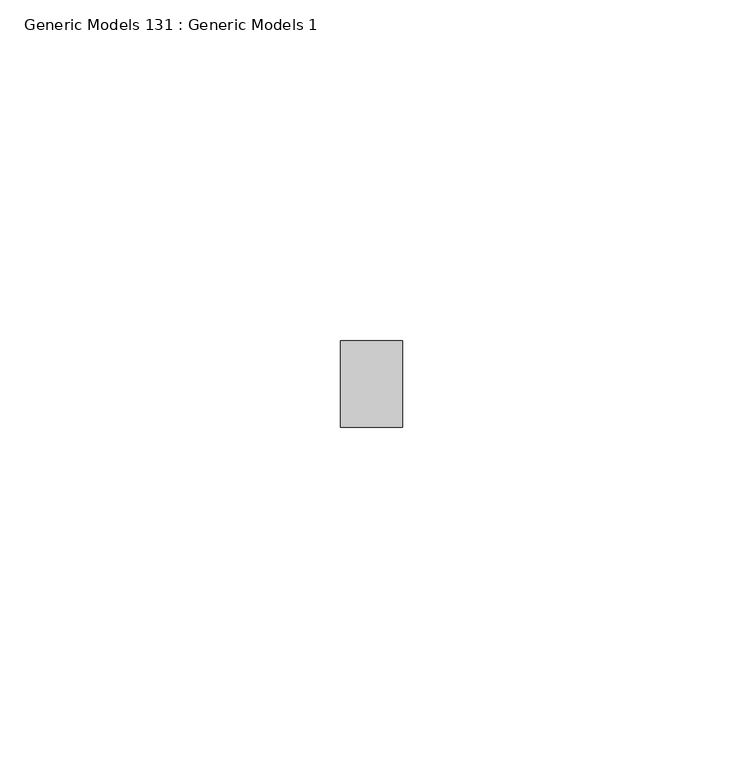
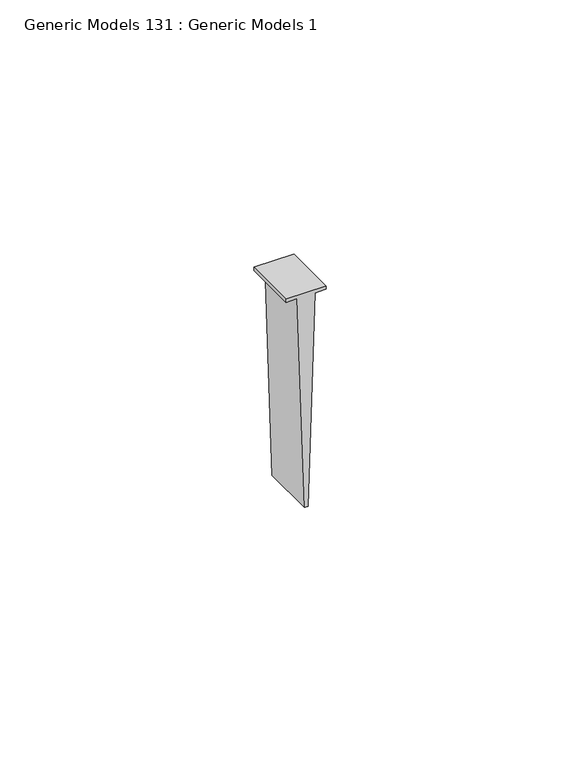
"""IFC4 building model written with IfcOpenShell, lengths in millimetres: proxy geometry, Generic Models 131 : Generic Models 1."""

import ifcopenshell
import ifcopenshell.guid

model = None  # the IFC model being written
_history = None  # IfcOwnerHistory: only IFC2X3 demands one
_inside = {}  # id of a spatial element -> (the spatial element, [elements in it])
_under = {}  # id of a project, library or spatial element -> (it, [spatial elements below it])
_declared = {}  # id of a project -> (the project, [libraries it declares])
_typed = {}  # id of a type object -> (the type object, [elements of that type])
_made_of = {}  # id of a material, layer set ... -> (it, [elements and type objects made of it])


def new_model(schema):
    """Start an empty IFC model of exactly this schema.

    Asked for "IFC4X3", IfcOpenShell would pick the latest addendum, in which some entities
    have other attributes; the version numbers below select the first issue.
    IFC2X3 requires an IfcOwnerHistory on every rooted entity: one is made here for all.
    """
    global model, _history
    if schema == "IFC4X3":
        model = ifcopenshell.file(schema_version=(4, 3, 0, 0))
    else:
        model = ifcopenshell.file(schema=schema)
    _inside.clear()
    _under.clear()
    _declared.clear()
    _typed.clear()
    _made_of.clear()
    _history = None
    if model.schema == "IFC2X3":
        org = make("IfcOrganization", Name="unknown")
        user = make(
            "IfcPersonAndOrganization",
            ThePerson=make("IfcPerson", FamilyName="unknown"),
            TheOrganization=org,
        )
        app = make(
            "IfcApplication",
            ApplicationDeveloper=org,
            Version="unknown",
            ApplicationFullName="unknown",
            ApplicationIdentifier="unknown",
        )
        _history = make(
            "IfcOwnerHistory",
            OwningUser=user,
            OwningApplication=app,
            ChangeAction="ADDED",
            CreationDate=0,
        )
    return model


def make(cls, **values):
    """One entity of the class cls with the attributes given. An attribute that is None is left unset."""
    return model.create_entity(
        cls, **{name: value for name, value in values.items() if value is not None}
    )


def rooted(cls, **values):
    """An entity with a GlobalId (a new one), such as an element, a storey or a relation."""
    return make(cls, GlobalId=ifcopenshell.guid.new(), OwnerHistory=_history, **values)


def si_unit(unit_type, name, prefix=None):
    """IfcSIUnit, for example si_unit("LENGTHUNIT", "METRE", prefix="MILLI")."""
    return make("IfcSIUnit", UnitType=unit_type, Prefix=prefix, Name=name)


def assignment(units):
    """IfcUnitAssignment: the units of a project."""
    return None if units is None else make("IfcUnitAssignment", Units=units)


def point(xyz):
    """IfcCartesianPoint."""
    return None if xyz is None else make("IfcCartesianPoint", Coordinates=xyz)


def direction(xyz):
    """IfcDirection."""
    return None if xyz is None else make("IfcDirection", DirectionRatios=xyz)


def frame(location, z_axis=None, x_axis=None):
    """IfcAxis2Placement3D, a coordinate frame: its origin and axes. An axis left out is left unset."""
    return make(
        "IfcAxis2Placement3D",
        Location=point(location),
        Axis=direction(z_axis),
        RefDirection=direction(x_axis),
    )


def origin():
    """The frame at (0, 0, 0) with its axes left unset."""
    return frame((0.0, 0.0, 0.0))


def place(relative_to, where):
    """IfcLocalPlacement: puts the frame where relative to a parent placement (None: the world)."""
    return make(
        "IfcLocalPlacement", PlacementRelTo=relative_to, RelativePlacement=where
    )


def context(
    kind, dimensions, precision=None, world=None, true_north=None, identifier=None
):
    """IfcGeometricRepresentationContext, for example the 3D "Model" context."""
    return make(
        "IfcGeometricRepresentationContext",
        ContextIdentifier=identifier,
        ContextType=kind,
        CoordinateSpaceDimension=dimensions,
        Precision=precision,
        WorldCoordinateSystem=world,
        TrueNorth=true_north,
    )


def project(units=None, contexts=None):
    """IfcProject with its units and contexts."""
    return rooted(
        "IfcProject",
        Name="project",
        RepresentationContexts=contexts,
        UnitsInContext=assignment(units),
    )


def spatial(cls, under=None, at=None, **own):
    """A site, building, storey or space (cls), placed at a placement, below another one or the project."""
    s = rooted(cls, ObjectPlacement=at, **own)
    if under is not None:
        _under.setdefault(under.id(), (under, []))[1].append(s)
    return s


def polyline(points):
    """IfcPolyline through the points."""
    return make("IfcPolyline", Points=[point(p) for p in points])


def outline(outer, holes=None, kind="AREA"):
    """IfcArbitraryClosedProfileDef: a profile drawn as a closed curve; with holes, ...WithVoids."""
    if holes is None:
        return make("IfcArbitraryClosedProfileDef", ProfileType=kind, OuterCurve=outer)
    return make(
        "IfcArbitraryProfileDefWithVoids",
        ProfileType=kind,
        OuterCurve=outer,
        InnerCurves=holes,
    )


def extrude(swept, where, along, depth):
    """IfcExtrudedAreaSolid: the profile swept, set in the frame where, extruded along a direction by depth."""
    return make(
        "IfcExtrudedAreaSolid",
        SweptArea=swept,
        Position=where,
        ExtrudedDirection=direction(along),
        Depth=depth,
    )


def shape(context_of_items, identifier, shape_type, items):
    """IfcShapeRepresentation: the items that make up one representation, for example the "Body"."""
    return make(
        "IfcShapeRepresentation",
        ContextOfItems=context_of_items,
        RepresentationIdentifier=identifier,
        RepresentationType=shape_type,
        Items=items,
    )


def source(mapping_origin, context_of_items, identifier, shape_type, items):
    """IfcRepresentationMap: a shape defined once, which mapped items show again and again."""
    return make(
        "IfcRepresentationMap",
        MappingOrigin=mapping_origin,
        MappedRepresentation=shape(context_of_items, identifier, shape_type, items),
    )


def transform(
    local_origin,
    x_axis=None,
    y_axis=None,
    z_axis=None,
    scale=None,
    scale2=None,
    scale3=None,
    uniform=True,
):
    """IfcCartesianTransformationOperator3D, or its non-uniform kind. x_axis, y_axis, z_axis: its Axis1, 2, 3."""
    if uniform:
        return make(
            "IfcCartesianTransformationOperator3D",
            Axis1=direction(x_axis),
            Axis2=direction(y_axis),
            LocalOrigin=point(local_origin),
            Scale=scale,
            Axis3=direction(z_axis),
        )
    return make(
        "IfcCartesianTransformationOperator3DnonUniform",
        Axis1=direction(x_axis),
        Axis2=direction(y_axis),
        LocalOrigin=point(local_origin),
        Scale=scale,
        Axis3=direction(z_axis),
        Scale2=scale2,
        Scale3=scale3,
    )


def mapped(mapping_source, mapping_target):
    """IfcMappedItem: shows the shape of a source again, moved by a transform."""
    return make(
        "IfcMappedItem", MappingSource=mapping_source, MappingTarget=mapping_target
    )


def made_of(thing, what):
    """Note that an element or type object is made of a material, layer set ...; save() writes the relation."""
    if what is not None:
        _made_of.setdefault(what.id(), (what, []))[1].append(thing)
    return thing


def element(
    cls,
    number,
    at=None,
    inside=None,
    cuts=None,
    type_object=None,
    material=None,
    context=None,
    identifier="Body",
    shape_type=None,
    held_by="IfcProductDefinitionShape",
    body=None,
    shapes=None,
    **own,
):
    """One element of the class cls, such as IfcWall. Its Tag is "e" and its number.

    at: its placement. inside: the storey or other place that contains it. cuts: it is an
    opening in that element (IfcRelVoidsElement). A single representation is given by context,
    identifier, shape_type and body (its items); several are given by shapes. held_by: the class
    of the entity that holds the representations. save() writes the other relations.
    """
    e = rooted(cls, Tag="e%d" % number, ObjectPlacement=at, **own)
    if body is not None:
        shapes = [shape(context, identifier, shape_type, body)]
    if shapes is not None:
        e.Representation = make(held_by, Representations=shapes)
    if inside is not None:
        _inside.setdefault(inside.id(), (inside, []))[1].append(e)
    if cuts is not None:
        rooted(
            "IfcRelVoidsElement", RelatingBuildingElement=cuts, RelatedOpeningElement=e
        )
    if type_object is not None:
        _typed.setdefault(type_object.id(), (type_object, []))[1].append(e)
    return made_of(e, material)


def aggregate(whole, parts):
    """IfcRelAggregates: a whole, such as a stair, and the parts it consists of."""
    return rooted("IfcRelAggregates", RelatingObject=whole, RelatedObjects=parts)


def save(model, path):
    """Write the relations noted so far, then the file.

    IfcRelAggregates (storeys below a building ...), IfcRelContainedInSpatialStructure (elements
    in a storey), IfcRelDefinesByType, IfcRelAssociatesMaterial and IfcRelDeclares: one each for
    every whole, place, type object, material and project.
    """
    for whole, parts in _under.values():
        aggregate(whole, parts)
    for where, things in _inside.values():
        rooted(
            "IfcRelContainedInSpatialStructure",
            RelatedElements=things,
            RelatingStructure=where,
        )
    for kind, things in _typed.values():
        rooted("IfcRelDefinesByType", RelatedObjects=things, RelatingType=kind)
    for what, things in _made_of.values():
        rooted("IfcRelAssociatesMaterial", RelatedObjects=things, RelatingMaterial=what)
    for by, libraries in _declared.values():
        rooted("IfcRelDeclares", RelatingContext=by, RelatedDefinitions=libraries)
    model.write(path)


def generic_models_131_generic_models_1_dfd9233a(model_context):
    return source(origin(), model_context, "Body", "SweptSolid", [
        extrude(outline(polyline([(-223.594817, 46885.2894531), (-224.388567, 46885.2894531), (-224.388567, 46887.8393167), (-275.188567, 46889.4367058), (-275.188567, 46890.2354003), (-224.388567, 46891.8327895), (-224.388567, 46894.3826531), (-223.594817, 46894.3826531), (-223.594817, 46885.2894531)])), frame((0.0, 565.15, 0.0), z_axis=(0.0, 1.0, 0.0), x_axis=(0.0, 0.0, 1.0)), (0.0, 0.0, 1.0), 12.7),
    ])


if __name__ == "__main__":
    model = new_model("IFC4")
    model_context = context("Model", 3, world=origin())
    ifc_project = project(units=[si_unit("LENGTHUNIT", "METRE", prefix="MILLI")], contexts=[model_context])
    site = spatial("IfcSite", under=ifc_project)
    building = spatial("IfcBuilding", under=site)
    placement = place(None, origin())
    generic_models_131_generic_models_1_shape = generic_models_131_generic_models_1_dfd9233a(model_context)
    element("IfcBuildingElementProxy", 1, Name="Generic Models 131 : Generic Models 1", ObjectType="Generic Models 131 : Generic Models 1", at=placement, inside=building, context=model_context, shape_type="MappedRepresentation", body=[
        mapped(generic_models_131_generic_models_1_shape, transform((0.0, 0.0, 0.0), x_axis=(1.0, 0.0, 0.0), y_axis=(0.0, 1.0, 0.0), z_axis=(0.0, 0.0, 1.0))),
    ])
    save(model, "model.ifc")

# Revit data of these elements
# Element 1 (IfcBuildingElementProxy, "Generic Models 131 : Generic Models 1")
#   Materials on its faces: "METAL RUNNER CHANNEL; FASTEN @ 24\" O.C."
# Materials
#   "METAL RUNNER CHANNEL; FASTEN @ 24\" O.C.": class "Unassigned", colour RGB 210 209 208, transparency 0, Keynote = "M05121300.02", Cost = 0
